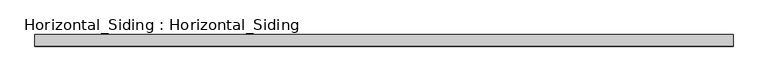
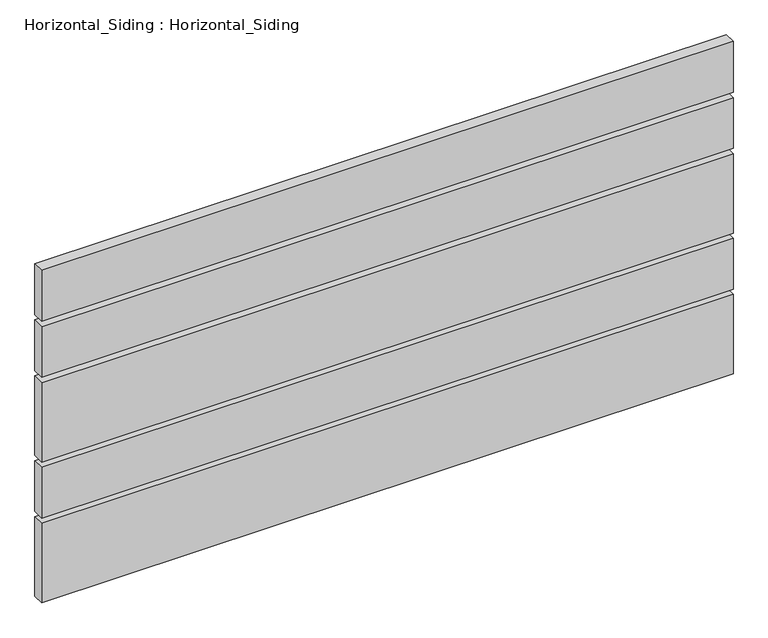
"""IFC4 building model written with IfcOpenShell, lengths in millimetres: plate geometry, Horizontal_Siding : Horizontal_Siding."""

from ifc_helpers import new_model, si_unit, frame, origin, place, context, project, spatial, polyline, outline, extrude, source, transform, mapped, element, save


def horizontal_siding_horizontal_siding_88204455(model_context):
    return source(origin(), model_context, "Body", "SweptSolid", [
        extrude(outline(polyline([(574.6750002, 19.05), (574.6750002, 0.0), (-574.6750002, 0.0), (-574.6750002, 19.05), (574.6750002, 19.05)])), frame((0.0, 0.0, 9.525), z_axis=(0.0, 0.0, 1.0), x_axis=(1.0, 0.0, 0.0)), (0.0, 0.0, 1.0), 139.7),
        extrude(outline(polyline([(574.6750002, 19.05), (574.6750002, 0.0), (-574.6750002, 0.0), (-574.6750002, 19.05), (574.6750002, 19.05)])), frame((0.0, 0.0, 158.75), z_axis=(0.0, 0.0, 1.0), x_axis=(1.0, 0.0, 0.0)), (0.0, 0.0, 1.0), 88.9),
        extrude(outline(polyline([(574.6750002, 19.05), (574.6750002, 0.0), (-574.6750002, 0.0), (-574.6750002, 19.05), (574.6750002, 19.05)])), frame((0.0, 0.0, 257.175), z_axis=(0.0, 0.0, 1.0), x_axis=(1.0, 0.0, 0.0)), (0.0, 0.0, 1.0), 139.7),
        extrude(outline(polyline([(574.6750002, 19.05), (574.6750002, 0.0), (-574.6750002, 0.0), (-574.6750002, 19.05), (574.6750002, 19.05)])), frame((0.0, 0.0, 406.4), z_axis=(0.0, 0.0, 1.0), x_axis=(1.0, 0.0, 0.0)), (0.0, 0.0, 1.0), 88.9),
        extrude(outline(polyline([(574.6750002, 19.05), (574.6750002, 0.0), (-574.6750002, 0.0), (-574.6750002, 19.05), (574.6750002, 19.05)])), frame((0.0, 0.0, 504.825), z_axis=(0.0, 0.0, 1.0), x_axis=(1.0, 0.0, 0.0)), (0.0, 0.0, 1.0), 88.9),
    ])


if __name__ == "__main__":
    model = new_model("IFC4")
    model_context = context("Model", 3, world=origin())
    ifc_project = project(units=[si_unit("LENGTHUNIT", "METRE", prefix="MILLI")], contexts=[model_context])
    site = spatial("IfcSite", under=ifc_project)
    building = spatial("IfcBuilding", under=site)
    placement = place(None, origin())
    horizontal_siding_horizontal_siding_shape = horizontal_siding_horizontal_siding_88204455(model_context)
    element("IfcPlate", 1, ObjectType="Horizontal_Siding : Horizontal_Siding", at=placement, inside=building, context=model_context, shape_type="MappedRepresentation", body=[
        mapped(horizontal_siding_horizontal_siding_shape, transform((0.0, 0.0, 0.0), x_axis=(1.0, 0.0, 0.0), y_axis=(0.0, 1.0, 0.0), z_axis=(0.0, 0.0, 1.0))),
    ])
    save(model, "model.ifc")

# Revit data of these elements
# Type "Horizontal_Siding : Horizontal_Siding"
#   Type Mark = "OUT"
#   Analytic Construction = "<None>"
#   extend = 0' - 2 3/4"
#   Width_2 = 0' - 3 1/2"
#   Width_1 = 0' - 5 1/2"
#   Gap = 0' - 0 3/8"
#   Plank Material = EXISTING HORZ. (1X4 & 1X6) WOOD SIDING (UNGROOVED PROFILE)
# Element 1 (IfcPlate, "Horizontal_Siding : Horizontal_Siding")
#   Materials on its faces: "EXISTING HORZ. (1X4 & 1X6) WOOD SIDING (UNGROOVED PROFILE)"
# Materials
#   "EXISTING HORZ. (1X4 & 1X6) WOOD SIDING (UNGROOVED PROFILE)": class "Wood", colour RGB 164 134 123, transparency 0, Description = "Pinus Echinata", Cost = 0
